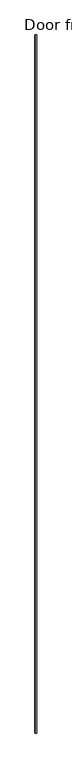
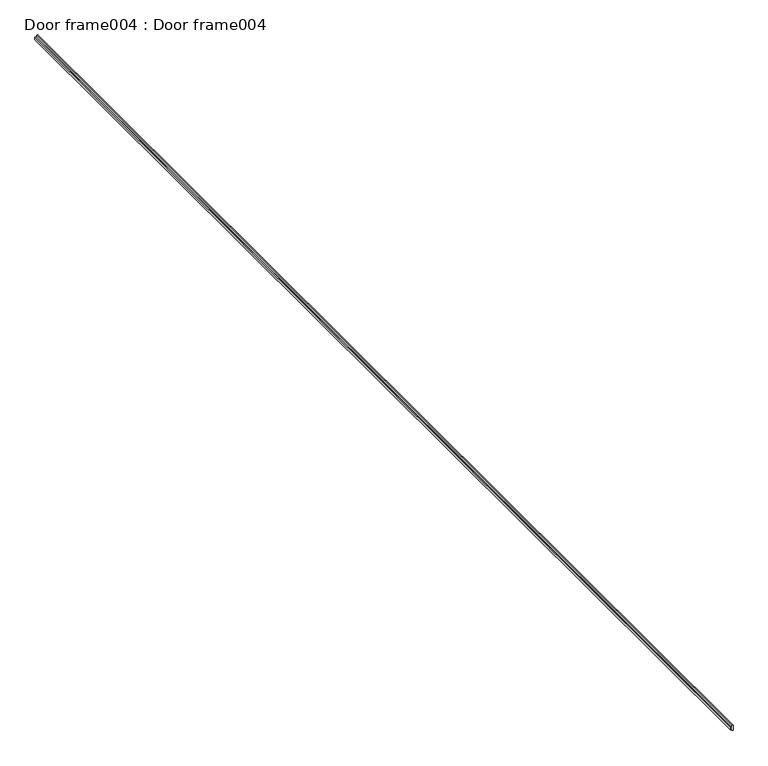
"""IFC4 building model written with IfcOpenShell, lengths in millimetres: proxy geometry, Door frame004 : Door frame004."""

import ifcopenshell
import ifcopenshell.guid

model = None  # the IFC model being written
_history = None  # IfcOwnerHistory: only IFC2X3 demands one
_inside = {}  # id of a spatial element -> (the spatial element, [elements in it])
_under = {}  # id of a project, library or spatial element -> (it, [spatial elements below it])
_declared = {}  # id of a project -> (the project, [libraries it declares])
_typed = {}  # id of a type object -> (the type object, [elements of that type])
_made_of = {}  # id of a material, layer set ... -> (it, [elements and type objects made of it])


def new_model(schema):
    """Start an empty IFC model of exactly this schema.

    Asked for "IFC4X3", IfcOpenShell would pick the latest addendum, in which some entities
    have other attributes; the version numbers below select the first issue.
    IFC2X3 requires an IfcOwnerHistory on every rooted entity: one is made here for all.
    """
    global model, _history
    if schema == "IFC4X3":
        model = ifcopenshell.file(schema_version=(4, 3, 0, 0))
    else:
        model = ifcopenshell.file(schema=schema)
    _inside.clear()
    _under.clear()
    _declared.clear()
    _typed.clear()
    _made_of.clear()
    _history = None
    if model.schema == "IFC2X3":
        org = make("IfcOrganization", Name="unknown")
        user = make(
            "IfcPersonAndOrganization",
            ThePerson=make("IfcPerson", FamilyName="unknown"),
            TheOrganization=org,
        )
        app = make(
            "IfcApplication",
            ApplicationDeveloper=org,
            Version="unknown",
            ApplicationFullName="unknown",
            ApplicationIdentifier="unknown",
        )
        _history = make(
            "IfcOwnerHistory",
            OwningUser=user,
            OwningApplication=app,
            ChangeAction="ADDED",
            CreationDate=0,
        )
    return model


def make(cls, **values):
    """One entity of the class cls with the attributes given. An attribute that is None is left unset."""
    return model.create_entity(
        cls, **{name: value for name, value in values.items() if value is not None}
    )


def rooted(cls, **values):
    """An entity with a GlobalId (a new one), such as an element, a storey or a relation."""
    return make(cls, GlobalId=ifcopenshell.guid.new(), OwnerHistory=_history, **values)


def si_unit(unit_type, name, prefix=None):
    """IfcSIUnit, for example si_unit("LENGTHUNIT", "METRE", prefix="MILLI")."""
    return make("IfcSIUnit", UnitType=unit_type, Prefix=prefix, Name=name)


def assignment(units):
    """IfcUnitAssignment: the units of a project."""
    return None if units is None else make("IfcUnitAssignment", Units=units)


def point(xyz):
    """IfcCartesianPoint."""
    return None if xyz is None else make("IfcCartesianPoint", Coordinates=xyz)


def direction(xyz):
    """IfcDirection."""
    return None if xyz is None else make("IfcDirection", DirectionRatios=xyz)


def frame(location, z_axis=None, x_axis=None):
    """IfcAxis2Placement3D, a coordinate frame: its origin and axes. An axis left out is left unset."""
    return make(
        "IfcAxis2Placement3D",
        Location=point(location),
        Axis=direction(z_axis),
        RefDirection=direction(x_axis),
    )


def origin():
    """The frame at (0, 0, 0) with its axes left unset."""
    return frame((0.0, 0.0, 0.0))


def place(relative_to, where):
    """IfcLocalPlacement: puts the frame where relative to a parent placement (None: the world)."""
    return make(
        "IfcLocalPlacement", PlacementRelTo=relative_to, RelativePlacement=where
    )


def context(
    kind, dimensions, precision=None, world=None, true_north=None, identifier=None
):
    """IfcGeometricRepresentationContext, for example the 3D "Model" context."""
    return make(
        "IfcGeometricRepresentationContext",
        ContextIdentifier=identifier,
        ContextType=kind,
        CoordinateSpaceDimension=dimensions,
        Precision=precision,
        WorldCoordinateSystem=world,
        TrueNorth=true_north,
    )


def project(units=None, contexts=None):
    """IfcProject with its units and contexts."""
    return rooted(
        "IfcProject",
        Name="project",
        RepresentationContexts=contexts,
        UnitsInContext=assignment(units),
    )


def spatial(cls, under=None, at=None, **own):
    """A site, building, storey or space (cls), placed at a placement, below another one or the project."""
    s = rooted(cls, ObjectPlacement=at, **own)
    if under is not None:
        _under.setdefault(under.id(), (under, []))[1].append(s)
    return s


def polyline(points):
    """IfcPolyline through the points."""
    return make("IfcPolyline", Points=[point(p) for p in points])


def outline(outer, holes=None, kind="AREA"):
    """IfcArbitraryClosedProfileDef: a profile drawn as a closed curve; with holes, ...WithVoids."""
    if holes is None:
        return make("IfcArbitraryClosedProfileDef", ProfileType=kind, OuterCurve=outer)
    return make(
        "IfcArbitraryProfileDefWithVoids",
        ProfileType=kind,
        OuterCurve=outer,
        InnerCurves=holes,
    )


def extrude(swept, where, along, depth):
    """IfcExtrudedAreaSolid: the profile swept, set in the frame where, extruded along a direction by depth."""
    return make(
        "IfcExtrudedAreaSolid",
        SweptArea=swept,
        Position=where,
        ExtrudedDirection=direction(along),
        Depth=depth,
    )


def shape(context_of_items, identifier, shape_type, items):
    """IfcShapeRepresentation: the items that make up one representation, for example the "Body"."""
    return make(
        "IfcShapeRepresentation",
        ContextOfItems=context_of_items,
        RepresentationIdentifier=identifier,
        RepresentationType=shape_type,
        Items=items,
    )


def source(mapping_origin, context_of_items, identifier, shape_type, items):
    """IfcRepresentationMap: a shape defined once, which mapped items show again and again."""
    return make(
        "IfcRepresentationMap",
        MappingOrigin=mapping_origin,
        MappedRepresentation=shape(context_of_items, identifier, shape_type, items),
    )


def transform(
    local_origin,
    x_axis=None,
    y_axis=None,
    z_axis=None,
    scale=None,
    scale2=None,
    scale3=None,
    uniform=True,
):
    """IfcCartesianTransformationOperator3D, or its non-uniform kind. x_axis, y_axis, z_axis: its Axis1, 2, 3."""
    if uniform:
        return make(
            "IfcCartesianTransformationOperator3D",
            Axis1=direction(x_axis),
            Axis2=direction(y_axis),
            LocalOrigin=point(local_origin),
            Scale=scale,
            Axis3=direction(z_axis),
        )
    return make(
        "IfcCartesianTransformationOperator3DnonUniform",
        Axis1=direction(x_axis),
        Axis2=direction(y_axis),
        LocalOrigin=point(local_origin),
        Scale=scale,
        Axis3=direction(z_axis),
        Scale2=scale2,
        Scale3=scale3,
    )


def mapped(mapping_source, mapping_target):
    """IfcMappedItem: shows the shape of a source again, moved by a transform."""
    return make(
        "IfcMappedItem", MappingSource=mapping_source, MappingTarget=mapping_target
    )


def made_of(thing, what):
    """Note that an element or type object is made of a material, layer set ...; save() writes the relation."""
    if what is not None:
        _made_of.setdefault(what.id(), (what, []))[1].append(thing)
    return thing


def element(
    cls,
    number,
    at=None,
    inside=None,
    cuts=None,
    type_object=None,
    material=None,
    context=None,
    identifier="Body",
    shape_type=None,
    held_by="IfcProductDefinitionShape",
    body=None,
    shapes=None,
    **own,
):
    """One element of the class cls, such as IfcWall. Its Tag is "e" and its number.

    at: its placement. inside: the storey or other place that contains it. cuts: it is an
    opening in that element (IfcRelVoidsElement). A single representation is given by context,
    identifier, shape_type and body (its items); several are given by shapes. held_by: the class
    of the entity that holds the representations. save() writes the other relations.
    """
    e = rooted(cls, Tag="e%d" % number, ObjectPlacement=at, **own)
    if body is not None:
        shapes = [shape(context, identifier, shape_type, body)]
    if shapes is not None:
        e.Representation = make(held_by, Representations=shapes)
    if inside is not None:
        _inside.setdefault(inside.id(), (inside, []))[1].append(e)
    if cuts is not None:
        rooted(
            "IfcRelVoidsElement", RelatingBuildingElement=cuts, RelatedOpeningElement=e
        )
    if type_object is not None:
        _typed.setdefault(type_object.id(), (type_object, []))[1].append(e)
    return made_of(e, material)


def aggregate(whole, parts):
    """IfcRelAggregates: a whole, such as a stair, and the parts it consists of."""
    return rooted("IfcRelAggregates", RelatingObject=whole, RelatedObjects=parts)


def save(model, path):
    """Write the relations noted so far, then the file.

    IfcRelAggregates (storeys below a building ...), IfcRelContainedInSpatialStructure (elements
    in a storey), IfcRelDefinesByType, IfcRelAssociatesMaterial and IfcRelDeclares: one each for
    every whole, place, type object, material and project.
    """
    for whole, parts in _under.values():
        aggregate(whole, parts)
    for where, things in _inside.values():
        rooted(
            "IfcRelContainedInSpatialStructure",
            RelatedElements=things,
            RelatingStructure=where,
        )
    for kind, things in _typed.values():
        rooted("IfcRelDefinesByType", RelatedObjects=things, RelatingType=kind)
    for what, things in _made_of.values():
        rooted("IfcRelAssociatesMaterial", RelatedObjects=things, RelatingMaterial=what)
    for by, libraries in _declared.values():
        rooted("IfcRelDeclares", RelatingContext=by, RelatedDefinitions=libraries)
    model.write(path)


def door_frame004_door_frame004_03d84ab6(model_context):
    return source(origin(), model_context, "Body", "SweptSolid", [
        extrude(outline(polyline([(36685.3750947, 15525.9592515), (36685.3750947, 15524.8924515), (36680.8030947, 15524.8924515), (36680.8030947, 15525.9592515), (36682.2000947, 15525.9592515), (36682.2000947, 15527.7372515), (36678.7014343, 15527.7372515), (36678.7014343, 15529.9292246), (36687.4772673, 15529.9292246), (36687.4772673, 15527.7373022), (36683.9780947, 15527.7373022), (36683.9780947, 15525.9592515), (36685.3750947, 15525.9592515)])), frame((0.0, -1052.8906567, 0.0), z_axis=(0.0, 1.0, 0.0), x_axis=(0.0, 0.0, 1.0)), (0.0, 0.0, 1.0), 1999.85),
    ])


if __name__ == "__main__":
    model = new_model("IFC4")
    model_context = context("Model", 3, world=origin())
    ifc_project = project(units=[si_unit("LENGTHUNIT", "METRE", prefix="MILLI")], contexts=[model_context])
    site = spatial("IfcSite", under=ifc_project)
    building = spatial("IfcBuilding", under=site)
    placement = place(None, origin())
    door_frame004_door_frame004_shape = door_frame004_door_frame004_03d84ab6(model_context)
    element("IfcBuildingElementProxy", 1, Name="Door frame004 : Door frame004", ObjectType="Door frame004 : Door frame004", at=placement, inside=building, context=model_context, shape_type="MappedRepresentation", body=[
        mapped(door_frame004_door_frame004_shape, transform((0.0, 0.0, 0.0), x_axis=(1.0, 0.0, 0.0), y_axis=(0.0, 1.0, 0.0), z_axis=(0.0, 0.0, 1.0))),
    ])
    save(model, "model.ifc")

# Revit data of these elements
# Type "Door frame004 : Door frame004"
#   NameOverride = "Door frame004"
# Element 1 (IfcBuildingElementProxy, "Door frame004 : Door frame004")
#   Materials on its faces: "FLEETWOOD SERIES T-3200 SINGLE SWING DOOR FRAME"
# Materials
#   "FLEETWOOD SERIES T-3200 SINGLE SWING DOOR FRAME": class "Unassigned", colour RGB 128 128 128, transparency 0, Cost = 0
